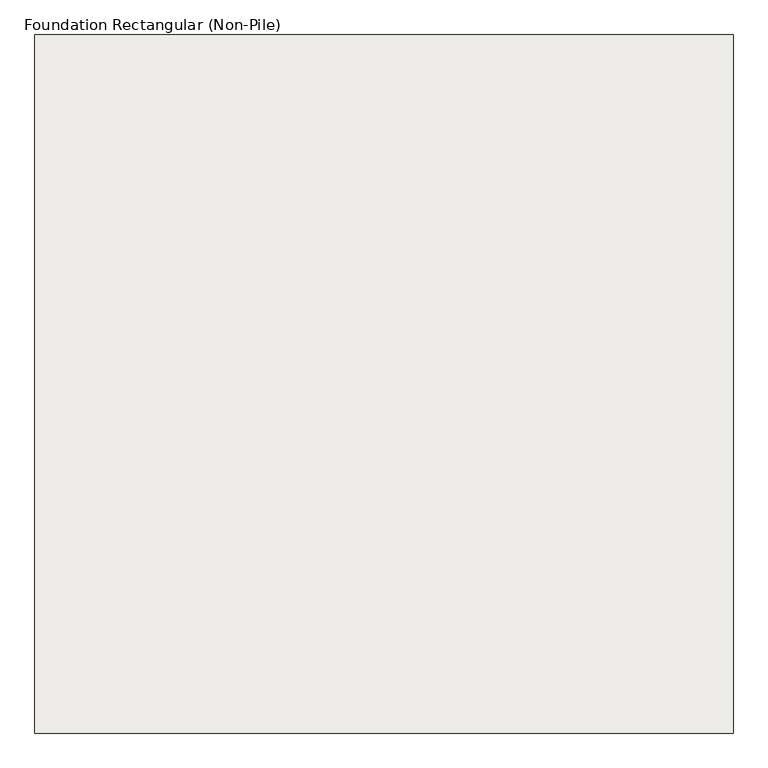
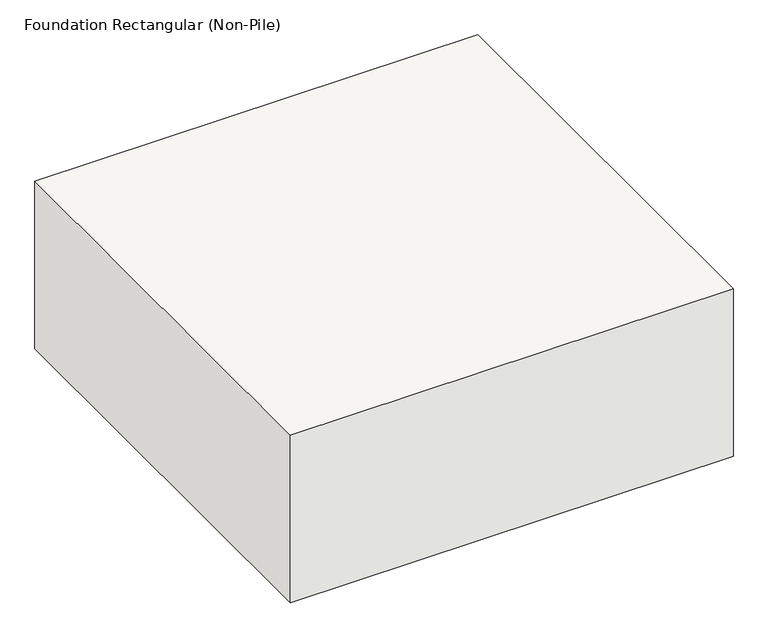
"""IFC4 building model written with IfcOpenShell, lengths in millimetres: slab geometry, Foundation Rectangular (Non-Pile) : H_SF_AR_S18_W1250xL1250xT500_Bitumen_F2."""

from ifc_helpers import new_model, si_unit, frame, origin, place, context, project, spatial, polyline, outline, extrude, source, transform, mapped, element, save


def foundation_rectangular_non_pile_17b72d6a(model_context):
    return source(origin(), model_context, "Body", "SweptSolid", [
        extrude(outline(polyline([(625.0, 625.0), (625.0, -625.0), (-625.0, -625.0), (-625.0, 625.0), (625.0, 625.0)])), frame((0.0, 0.0, -500.0), z_axis=(0.0, 0.0, 1.0), x_axis=(1.0, 0.0, 0.0)), (0.0, 0.0, 1.0), 500.0),
    ])


if __name__ == "__main__":
    model = new_model("IFC4")
    model_context = context("Model", 3, world=origin())
    ifc_project = project(units=[si_unit("LENGTHUNIT", "METRE", prefix="MILLI")], contexts=[model_context])
    site = spatial("IfcSite", under=ifc_project)
    building = spatial("IfcBuilding", under=site)
    placement = place(None, origin())
    foundation_rectangular_non_pile_shape = foundation_rectangular_non_pile_17b72d6a(model_context)
    element("IfcSlab", 1, ObjectType="Foundation Rectangular (Non-Pile) : H_SF_AR_S18_W1250xL1250xT500_Bitumen_F2", at=placement, inside=building, context=model_context, shape_type="MappedRepresentation", body=[
        mapped(foundation_rectangular_non_pile_shape, transform((0.0, 0.0, 0.0), x_axis=(1.0, 0.0, 0.0), y_axis=(0.0, 1.0, 0.0), z_axis=(0.0, 0.0, 1.0))),
    ])
    save(model, "model.ifc")

# Revit data of these elements
# Type "Foundation Rectangular (Non-Pile) : H_SF_AR_S18_W1250xL1250xT500_Bitumen_F2"
#   Type Comments = "UG"
#   Type Mark = "F2"
#   H_Q'ty Cal Type Tag = "SB-Q1"
#   H_WM Code_1 = "A03AF032-00022 |  | M3 | Concrete Work | Superstructure Work | Structural Concrete | Cement Type-1 | 25MPa ≤ F'c (Cylinder Strength) < 30MPa |  |  |  |  | A03AF032-00022 Concrete Work Superstructure Work Structural Concrete  Cement Type-1 25MPa ≤ F'c (Cylinder Strength) < 30MPa      |  F'c (Cylinder Strength) = 24MPa"
#   H_WM Code_2 = "A03AD037-00002 |  | TON | Concrete Work | Substructure Work | Rebar Work | Deformed Bar (Non-Coat.) | 400MPa<Fy≤470MPa |  |  |  |  | A03AD037-00002 Concrete Work Substructure Work Rebar Work Deformed Bar (Non-Coat.)  400MPa<Fy≤470MPa      | ASTM A615 GRADE 60 (Fy=420MPa)"
#   H_WM Code_3 = "A03AF036-00001 |  | M2 | Concrete Work | Superstructure Work | Form Work (1 time in use) | Flat Form | Dressed Lumber, Plywood or Steel Form(Wood Planks are not Allowed) incl. Chamfer |  |  |  | A03AF036-00001 Concrete Work Superstructure Work Form Work (1 time in use) Flat Form     Dressed Lumber, Plywood or Steel Form(Wood Planks are not Allowed) incl. Chamfer   |"
#   Top bar = "D25@300"
#   Description = "UG Shallow Foundation"
#   Bottom bar = "D20@300"
#   Width = 1250 mm
#   Length = 1250 mm
#   Foundation Thickness = 500 mm
#   Structural Material [instance default] = none
#   Assembly Code = ""
# Element 1 (IfcSlab, "Foundation Rectangular (Non-Pile) : H_SF_AR_S18_W1250xL1250xT500_Bitumen_F2")
#   Structural Material = 00_Concrete_Reinf. Conc.
#   Materials on its faces: "00_Concrete_Reinf. Conc."
# Materials
#   "00_Concrete_Reinf. Conc.": class "Concrete", colour RGB 176 176 176, transparency 0, Description = "Reinf. Conc.", Cost = 0, Image = Concrete.Cast-In-Place.Flat.Polished.Grey.jpg
